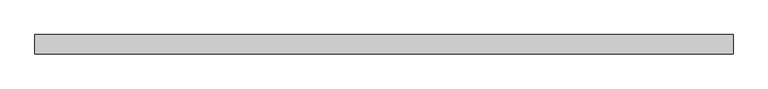
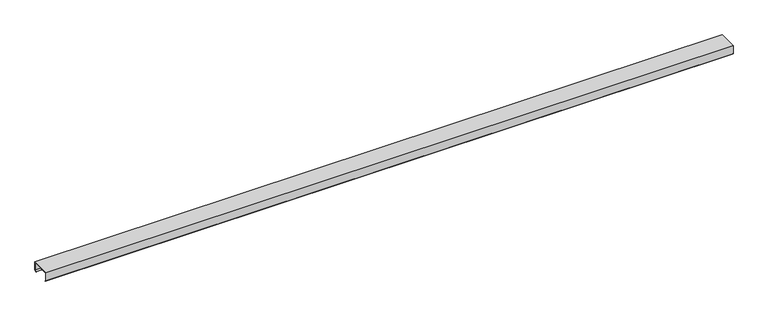
"""IFC4 building model written with IfcOpenShell, lengths in millimetres: proxy geometry, Generic Models 7:Generic Models 1:1:Generic Models 1:1 : Generic Models 7:Generic Models 1:337419:6 : Generic Models 7:Generic Models 1:1:Generic Models 1:1 : Generic Models 7:Generic Models 1:337419:306201."""

from ifc_helpers import new_model, si_unit, frame, origin, place, context, project, spatial, polyline, outline, extrude, source, transform, mapped, element, save


def generic_models_b1f3a948(model_context):
    return source(origin(), model_context, "Body", "SweptSolid", [
        extrude(outline(polyline([(-579000.6913841, 1309.4890625), (-578797.4913841, 1309.4890625), (-578797.4913841, 1220.5890625), (-578812.0845307, 1208.3439586), (-578813.8702751, 1210.4721258), (-578800.2695091, 1221.8845235), (-578800.2695091, 1306.7109375), (-578997.9132591, 1306.7109375), (-578997.9132591, 1221.8845235), (-578984.3124931, 1210.4721258), (-578986.0982375, 1208.3439586), (-579000.6913841, 1220.5890625), (-579000.6913841, 1309.4890625)])), frame((565582.1867239, 0.0, 0.0), z_axis=(1.0, 0.0, 0.0), x_axis=(0.0, 1.0, 0.0)), (0.0, 0.0, 1.0), 7315.2),
    ])


if __name__ == "__main__":
    model = new_model("IFC4")
    model_context = context("Model", 3, world=origin())
    ifc_project = project(units=[si_unit("LENGTHUNIT", "METRE", prefix="MILLI")], contexts=[model_context])
    site = spatial("IfcSite", under=ifc_project)
    building = spatial("IfcBuilding", under=site)
    placement = place(None, origin())
    generic_models_shape = generic_models_b1f3a948(model_context)
    element("IfcBuildingElementProxy", 1, Name="Generic Models 7:Generic Models 1:1:Generic Models 1:1 : Generic Models 7:Generic Models 1:337419:6 : Generic Models 7:Generic Models 1:1:Generic Models 1:1 : Generic Models 7:Generic Models 1:337419:306201", ObjectType="Generic Models 7:Generic Models 1:1:Generic Models 1:1 : Generic Models 7:Generic Models 1:337419:6 : Generic Models 7:Generic Models 1:1:Generic Models 1:1 : Generic Models 7:Generic Models 1:337419:306201", at=placement, inside=building, context=model_context, shape_type="MappedRepresentation", body=[
        mapped(generic_models_shape, transform((0.0, 0.0, 0.0), x_axis=(1.0, 0.0, 0.0), y_axis=(0.0, 1.0, 0.0), z_axis=(0.0, 0.0, 1.0))),
    ])
    save(model, "model.ifc")

# Revit data of these elements
# Type "Generic Models 7:Generic Models 1:1:Generic Models 1:1 : Generic Models 7:Generic Models 1:337419:6 : Generic Models 7:Generic Models 1:1:Generic Models 1:1 : Generic Models 7:Generic Models 1:337419:306201"
#   NameOverride = "Generic Models 7:Generic Models 1:1:Generic Models 1:1 : Generic Models 7:Generic Models 1:337419:306201"
#   ObjectTypeOverride = "Generic Models 1:1 : Generic Models 7:Generic Models 1:337419"
#   Reference = "Generic Models 1"
#   Tag = "306201"
# Element 1 (IfcBuildingElementProxy, "Generic Models 7:Generic Models 1:1:Generic Models 1:1 : Generic Models 7:Generic Models 1:337419:6 : Generic Models 7:Generic Models 1:1:Generic Models 1:1 : Generic Models 7:Generic Models 1:337419:306201")
#   Materials on its faces: "CEE' SECTION (8.0x3.5C - SEE STRUCT. DWGS)"
# Materials
#   "CEE' SECTION (8.0x3.5C - SEE STRUCT. DWGS)": class "Unassigned", colour RGB 210 209 208, transparency 0, Keynote = "M05121300.02", Cost = 0
